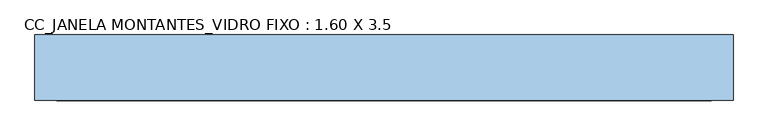
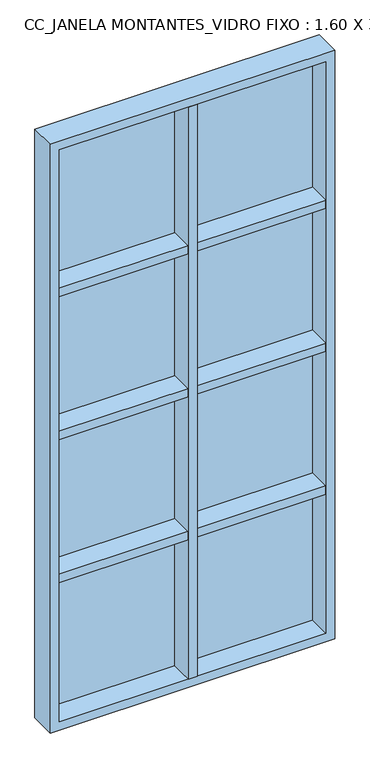
"""IFC4 building model written with IfcOpenShell, lengths in millimetres: window geometry, CC_JANELA MONTANTES_VIDRO FIXO : 1.60 X 3.5."""

import ifcopenshell
import ifcopenshell.guid

model = None  # the IFC model being written
_history = None  # IfcOwnerHistory: only IFC2X3 demands one
_inside = {}  # id of a spatial element -> (the spatial element, [elements in it])
_under = {}  # id of a project, library or spatial element -> (it, [spatial elements below it])
_declared = {}  # id of a project -> (the project, [libraries it declares])
_typed = {}  # id of a type object -> (the type object, [elements of that type])
_made_of = {}  # id of a material, layer set ... -> (it, [elements and type objects made of it])


def new_model(schema):
    """Start an empty IFC model of exactly this schema.

    Asked for "IFC4X3", IfcOpenShell would pick the latest addendum, in which some entities
    have other attributes; the version numbers below select the first issue.
    IFC2X3 requires an IfcOwnerHistory on every rooted entity: one is made here for all.
    """
    global model, _history
    if schema == "IFC4X3":
        model = ifcopenshell.file(schema_version=(4, 3, 0, 0))
    else:
        model = ifcopenshell.file(schema=schema)
    _inside.clear()
    _under.clear()
    _declared.clear()
    _typed.clear()
    _made_of.clear()
    _history = None
    if model.schema == "IFC2X3":
        org = make("IfcOrganization", Name="unknown")
        user = make(
            "IfcPersonAndOrganization",
            ThePerson=make("IfcPerson", FamilyName="unknown"),
            TheOrganization=org,
        )
        app = make(
            "IfcApplication",
            ApplicationDeveloper=org,
            Version="unknown",
            ApplicationFullName="unknown",
            ApplicationIdentifier="unknown",
        )
        _history = make(
            "IfcOwnerHistory",
            OwningUser=user,
            OwningApplication=app,
            ChangeAction="ADDED",
            CreationDate=0,
        )
    return model


def make(cls, **values):
    """One entity of the class cls with the attributes given. An attribute that is None is left unset."""
    return model.create_entity(
        cls, **{name: value for name, value in values.items() if value is not None}
    )


def rooted(cls, **values):
    """An entity with a GlobalId (a new one), such as an element, a storey or a relation."""
    return make(cls, GlobalId=ifcopenshell.guid.new(), OwnerHistory=_history, **values)


def si_unit(unit_type, name, prefix=None):
    """IfcSIUnit, for example si_unit("LENGTHUNIT", "METRE", prefix="MILLI")."""
    return make("IfcSIUnit", UnitType=unit_type, Prefix=prefix, Name=name)


def assignment(units):
    """IfcUnitAssignment: the units of a project."""
    return None if units is None else make("IfcUnitAssignment", Units=units)


def point(xyz):
    """IfcCartesianPoint."""
    return None if xyz is None else make("IfcCartesianPoint", Coordinates=xyz)


def direction(xyz):
    """IfcDirection."""
    return None if xyz is None else make("IfcDirection", DirectionRatios=xyz)


def frame(location, z_axis=None, x_axis=None):
    """IfcAxis2Placement3D, a coordinate frame: its origin and axes. An axis left out is left unset."""
    return make(
        "IfcAxis2Placement3D",
        Location=point(location),
        Axis=direction(z_axis),
        RefDirection=direction(x_axis),
    )


def origin():
    """The frame at (0, 0, 0) with its axes left unset."""
    return frame((0.0, 0.0, 0.0))


def place(relative_to, where):
    """IfcLocalPlacement: puts the frame where relative to a parent placement (None: the world)."""
    return make(
        "IfcLocalPlacement", PlacementRelTo=relative_to, RelativePlacement=where
    )


def context(
    kind, dimensions, precision=None, world=None, true_north=None, identifier=None
):
    """IfcGeometricRepresentationContext, for example the 3D "Model" context."""
    return make(
        "IfcGeometricRepresentationContext",
        ContextIdentifier=identifier,
        ContextType=kind,
        CoordinateSpaceDimension=dimensions,
        Precision=precision,
        WorldCoordinateSystem=world,
        TrueNorth=true_north,
    )


def project(units=None, contexts=None):
    """IfcProject with its units and contexts."""
    return rooted(
        "IfcProject",
        Name="project",
        RepresentationContexts=contexts,
        UnitsInContext=assignment(units),
    )


def spatial(cls, under=None, at=None, **own):
    """A site, building, storey or space (cls), placed at a placement, below another one or the project."""
    s = rooted(cls, ObjectPlacement=at, **own)
    if under is not None:
        _under.setdefault(under.id(), (under, []))[1].append(s)
    return s


def polyline(points):
    """IfcPolyline through the points."""
    return make("IfcPolyline", Points=[point(p) for p in points])


def outline(outer, holes=None, kind="AREA"):
    """IfcArbitraryClosedProfileDef: a profile drawn as a closed curve; with holes, ...WithVoids."""
    if holes is None:
        return make("IfcArbitraryClosedProfileDef", ProfileType=kind, OuterCurve=outer)
    return make(
        "IfcArbitraryProfileDefWithVoids",
        ProfileType=kind,
        OuterCurve=outer,
        InnerCurves=holes,
    )


def extrude(swept, where, along, depth):
    """IfcExtrudedAreaSolid: the profile swept, set in the frame where, extruded along a direction by depth."""
    return make(
        "IfcExtrudedAreaSolid",
        SweptArea=swept,
        Position=where,
        ExtrudedDirection=direction(along),
        Depth=depth,
    )


def shape(context_of_items, identifier, shape_type, items):
    """IfcShapeRepresentation: the items that make up one representation, for example the "Body"."""
    return make(
        "IfcShapeRepresentation",
        ContextOfItems=context_of_items,
        RepresentationIdentifier=identifier,
        RepresentationType=shape_type,
        Items=items,
    )


def source(mapping_origin, context_of_items, identifier, shape_type, items):
    """IfcRepresentationMap: a shape defined once, which mapped items show again and again."""
    return make(
        "IfcRepresentationMap",
        MappingOrigin=mapping_origin,
        MappedRepresentation=shape(context_of_items, identifier, shape_type, items),
    )


def transform(
    local_origin,
    x_axis=None,
    y_axis=None,
    z_axis=None,
    scale=None,
    scale2=None,
    scale3=None,
    uniform=True,
):
    """IfcCartesianTransformationOperator3D, or its non-uniform kind. x_axis, y_axis, z_axis: its Axis1, 2, 3."""
    if uniform:
        return make(
            "IfcCartesianTransformationOperator3D",
            Axis1=direction(x_axis),
            Axis2=direction(y_axis),
            LocalOrigin=point(local_origin),
            Scale=scale,
            Axis3=direction(z_axis),
        )
    return make(
        "IfcCartesianTransformationOperator3DnonUniform",
        Axis1=direction(x_axis),
        Axis2=direction(y_axis),
        LocalOrigin=point(local_origin),
        Scale=scale,
        Axis3=direction(z_axis),
        Scale2=scale2,
        Scale3=scale3,
    )


def mapped(mapping_source, mapping_target):
    """IfcMappedItem: shows the shape of a source again, moved by a transform."""
    return make(
        "IfcMappedItem", MappingSource=mapping_source, MappingTarget=mapping_target
    )


def made_of(thing, what):
    """Note that an element or type object is made of a material, layer set ...; save() writes the relation."""
    if what is not None:
        _made_of.setdefault(what.id(), (what, []))[1].append(thing)
    return thing


def element(
    cls,
    number,
    at=None,
    inside=None,
    cuts=None,
    type_object=None,
    material=None,
    context=None,
    identifier="Body",
    shape_type=None,
    held_by="IfcProductDefinitionShape",
    body=None,
    shapes=None,
    **own,
):
    """One element of the class cls, such as IfcWall. Its Tag is "e" and its number.

    at: its placement. inside: the storey or other place that contains it. cuts: it is an
    opening in that element (IfcRelVoidsElement). A single representation is given by context,
    identifier, shape_type and body (its items); several are given by shapes. held_by: the class
    of the entity that holds the representations. save() writes the other relations.
    """
    e = rooted(cls, Tag="e%d" % number, ObjectPlacement=at, **own)
    if body is not None:
        shapes = [shape(context, identifier, shape_type, body)]
    if shapes is not None:
        e.Representation = make(held_by, Representations=shapes)
    if inside is not None:
        _inside.setdefault(inside.id(), (inside, []))[1].append(e)
    if cuts is not None:
        rooted(
            "IfcRelVoidsElement", RelatingBuildingElement=cuts, RelatedOpeningElement=e
        )
    if type_object is not None:
        _typed.setdefault(type_object.id(), (type_object, []))[1].append(e)
    return made_of(e, material)


def aggregate(whole, parts):
    """IfcRelAggregates: a whole, such as a stair, and the parts it consists of."""
    return rooted("IfcRelAggregates", RelatingObject=whole, RelatedObjects=parts)


def save(model, path):
    """Write the relations noted so far, then the file.

    IfcRelAggregates (storeys below a building ...), IfcRelContainedInSpatialStructure (elements
    in a storey), IfcRelDefinesByType, IfcRelAssociatesMaterial and IfcRelDeclares: one each for
    every whole, place, type object, material and project.
    """
    for whole, parts in _under.values():
        aggregate(whole, parts)
    for where, things in _inside.values():
        rooted(
            "IfcRelContainedInSpatialStructure",
            RelatedElements=things,
            RelatingStructure=where,
        )
    for kind, things in _typed.values():
        rooted("IfcRelDefinesByType", RelatedObjects=things, RelatingType=kind)
    for what, things in _made_of.values():
        rooted("IfcRelAssociatesMaterial", RelatedObjects=things, RelatingMaterial=what)
    for by, libraries in _declared.values():
        rooted("IfcRelDeclares", RelatingContext=by, RelatedDefinitions=libraries)
    model.write(path)


def cc_janela_montantes_vidro_fixo_1_60_x_3_5_286e51ec(model_context):
    return source(origin(), model_context, "Body", "SweptSolid", [
        extrude(outline(polyline([(750.0, 97.5), (750.0, -47.5), (-750.0, -47.5), (-750.0, 97.5), (750.0, 97.5)])), frame((0.0, 0.0, 1875.0), z_axis=(0.0, 0.0, 1.0), x_axis=(1.0, 0.0, 0.0)), (0.0, 0.0, 1.0), 50.0),
        extrude(outline(polyline([(750.0, 97.5), (750.0, -47.5), (-750.0, -47.5), (-750.0, 97.5), (750.0, 97.5)])), frame((0.0, 0.0, 2725.0), z_axis=(0.0, 0.0, 1.0), x_axis=(1.0, 0.0, 0.0)), (0.0, 0.0, 1.0), 50.0),
        extrude(outline(polyline([(750.0, 97.5), (750.0, -47.5), (-750.0, -47.5), (-750.0, 97.5), (750.0, 97.5)])), frame((0.0, 0.0, 3575.0), z_axis=(0.0, 0.0, 1.0), x_axis=(1.0, 0.0, 0.0)), (0.0, 0.0, 1.0), 50.0),
        extrude(outline(polyline([(25.0, 100.0), (25.0, -50.0), (-25.0, -50.0), (-25.0, 100.0), (25.0, 100.0)])), frame((0.0, 0.0, 1050.0), z_axis=(0.0, 0.0, 1.0), x_axis=(1.0, 0.0, 0.0)), (0.0, 0.0, 1.0), 3400.0),
        extrude(outline(polyline([(4500.0, -800.0), (1000.0, -800.0), (1000.0, 800.0), (4500.0, 800.0), (4500.0, -800.0)]), holes=[polyline([(4450.0, -750.0), (4450.0, 750.0), (1050.0, 750.0), (1050.0, -750.0), (4450.0, -750.0)])]), frame((0.0, -50.0, 0.0), z_axis=(0.0, 1.0, 0.0), x_axis=(0.0, 0.0, 1.0)), (0.0, 0.0, 1.0), 150.0),
        extrude(outline(polyline([(750.0, 80.0), (-750.0, 80.0), (-750.0, 92.0), (750.0, 92.0), (750.0, 80.0)])), frame((0.0, 0.0, 1050.0), z_axis=(0.0, 0.0, 1.0), x_axis=(1.0, 0.0, 0.0)), (0.0, 0.0, 1.0), 3400.0),
    ])


if __name__ == "__main__":
    model = new_model("IFC4")
    model_context = context("Model", 3, world=origin())
    ifc_project = project(units=[si_unit("LENGTHUNIT", "METRE", prefix="MILLI")], contexts=[model_context])
    site = spatial("IfcSite", under=ifc_project)
    building = spatial("IfcBuilding", under=site)
    placement = place(None, origin())
    cc_janela_montantes_vidro_fixo_1_60_x_3_5_shape = cc_janela_montantes_vidro_fixo_1_60_x_3_5_286e51ec(model_context)
    element("IfcWindow", 1, ObjectType="CC_JANELA MONTANTES_VIDRO FIXO : 1.60 X 3.5", at=placement, inside=building, context=model_context, shape_type="MappedRepresentation", body=[
        mapped(cc_janela_montantes_vidro_fixo_1_60_x_3_5_shape, transform((0.0, 0.0, 0.0), x_axis=(1.0, 0.0, 0.0), y_axis=(0.0, 1.0, 0.0), z_axis=(0.0, 0.0, 1.0))),
    ])
    save(model, "model.ifc")

# Revit data of these elements
# Type "CC_JANELA MONTANTES_VIDRO FIXO : 1.60 X 3.5"
#   Type Mark = "J8"
#   Analytic Construction = "<Nenhum>"
#   Largura janela = 1.50 m
#   Espaçamento montantes verticais [instance default] = 0.75 m
#   Espaçamento montantes horizontais [instance default] = 0.85 m
#   Altura janela = 3.40 m
#   Height = 3.50 m
#   Altura-padrão do peitoril = 1.00 m
#   Width = 1.60 m
#   N verticais [instance default] = 2
#   N horizontais [instance default] = 3
#   N de montantes verticais [instance default] = 1
#   N de montantes horizontais [instance default] = 3
#   Montate vertical vários [instance default] = no
#   Montante vertical único [instance default] = yes
#   Montante horizontal único [instance default] = no
#   Montante horizontal vários [instance default] = yes
#   Tipo de vidro = .VIDRO
#   Material da esquadria = .ALUMÍNIO COM PINTURA ELETROSTÁTICA BRANCA
#   Wall Closure = (empty or 0)
# Element 1 (IfcWindow, "CC_JANELA MONTANTES_VIDRO FIXO : 1.60 X 3.5")
#   Materials on its faces: ".ALUMÍNIO COM PINTURA ELETROSTÁTICA BRANCA", ".VIDRO"
# Materials
#   ".VIDRO": class "Genérico", colour RGB 198 236 255, transparency 0.95, Cost = 0
#   ".ALUMÍNIO COM PINTURA ELETROSTÁTICA BRANCA": class "CC_METAIS", colour RGB 241 241 241, transparency 0, Cost = 0
